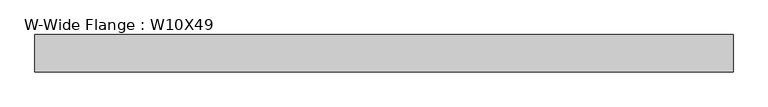
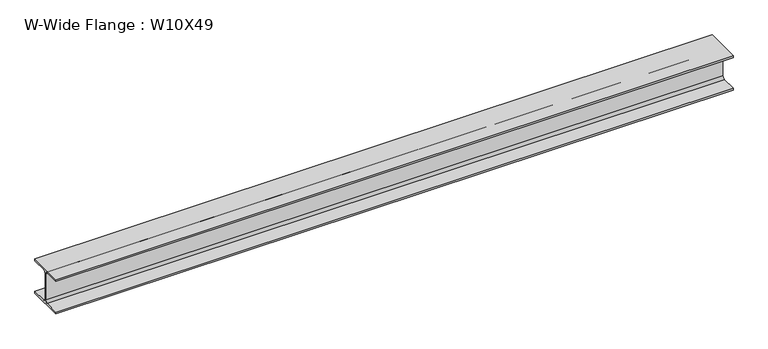
"""IFC4 building model written with IfcOpenShell, lengths in millimetres: beam geometry, W-Wide Flange : W10X49."""

from ifc_helpers import new_model, si_unit, point, frame, frame_2d, origin, place, context, project, spatial, polyline, circle_curve, trimmed, segment, composite_curve, outline, extrude, source, transform, mapped, element, save


def w_wide_flange_w10x49_8d358260(model_context):
    return source(origin(), model_context, "Body", "SweptSolid", [
        extrude(outline(composite_curve([segment(polyline([(127.0, -112.776), (127.0, -127.0), (-127.0, -127.0), (-127.0, -112.776), (-21.844, -112.776)]), True, "CONTINUOUS"), segment(trimmed(circle_curve(frame_2d((-21.844, -95.25)), 17.526), [point((-21.844, -112.776))], [point((-4.318, -95.25))], True, "CARTESIAN"), True, "CONTINUOUS"), segment(polyline([(-4.318, -95.25), (-4.318, 95.25)]), True, "CONTINUOUS"), segment(trimmed(circle_curve(frame_2d((-21.844, 95.25)), 17.526), [point((-4.318, 95.25))], [point((-21.844, 112.776))], True, "CARTESIAN"), True, "CONTINUOUS"), segment(polyline([(-21.844, 112.776), (-127.0, 112.776), (-127.0, 127.0), (127.0, 127.0), (127.0, 112.776), (21.844, 112.776)]), True, "CONTINUOUS"), segment(trimmed(circle_curve(frame_2d((21.844, 95.25)), 17.526), [point((21.844, 112.776))], [point((4.318, 95.25))], True, "CARTESIAN"), True, "CONTINUOUS"), segment(polyline([(4.318, 95.25), (4.318, -95.25)]), True, "CONTINUOUS"), segment(trimmed(circle_curve(frame_2d((21.844, -95.25)), 17.526), [point((4.318, -95.25))], [point((21.844, -112.776))], True, "CARTESIAN"), True, "CONTINUOUS"), segment(polyline([(21.844, -112.776), (127.0, -112.776)]), True, "CONTINUOUS")], self_intersect=False)), frame((-2340.5193905, 0.0, 0.0), z_axis=(1.0, 0.0, 0.0), x_axis=(0.0, 1.0, 0.0)), (0.0, 0.0, 1.0), 4725.406181),
    ])


if __name__ == "__main__":
    model = new_model("IFC4")
    model_context = context("Model", 3, world=origin())
    ifc_project = project(units=[si_unit("LENGTHUNIT", "METRE", prefix="MILLI")], contexts=[model_context])
    site = spatial("IfcSite", under=ifc_project)
    building = spatial("IfcBuilding", under=site)
    placement = place(None, origin())
    w_wide_flange_w10x49_shape = w_wide_flange_w10x49_8d358260(model_context)
    element("IfcBeam", 1, ObjectType="W-Wide Flange : W10X49", at=placement, inside=building, context=model_context, shape_type="MappedRepresentation", body=[
        mapped(w_wide_flange_w10x49_shape, transform((0.0, 0.0, 0.0), x_axis=(1.0, 0.0, 0.0), y_axis=(0.0, 1.0, 0.0), z_axis=(0.0, 0.0, 1.0))),
    ])
    save(model, "model.ifc")

# Revit data of these elements
# Type "W-Wide Flange : W10X49"
#   Assembly Code = "B10"
#   W = 49
#   Length [instance default] = 1524 mm
#   bf = 254 mm
#   d = 254 mm
#   k = 31.75 mm
#   k2 = 17.526 mm
#   tf = 14.224 mm
#   tw = 8.636 mm
#   A = 0.0092903 m²
#   Structural Material [instance default] = Steel ASTM A992
# Element 1 (IfcBeam, "W-Wide Flange : W10X49")
#   Structural Material = Aluminum, Anodized Red
#   Materials on its faces: "Aluminum, Anodized Red"
# Materials
#   "Steel ASTM A992": class "Metal", colour RGB 128 0 0, transparency 0, Description = "Structural steel 50ksi", Cost = 0
#   "Aluminum, Anodized Red": class "Metal", colour RGB 120 120 120, transparency 0, Description = "Anodized aluminum, red", Cost = 0
